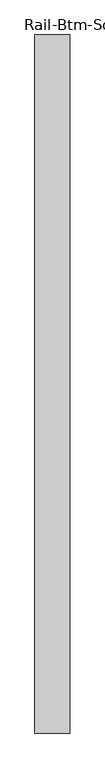
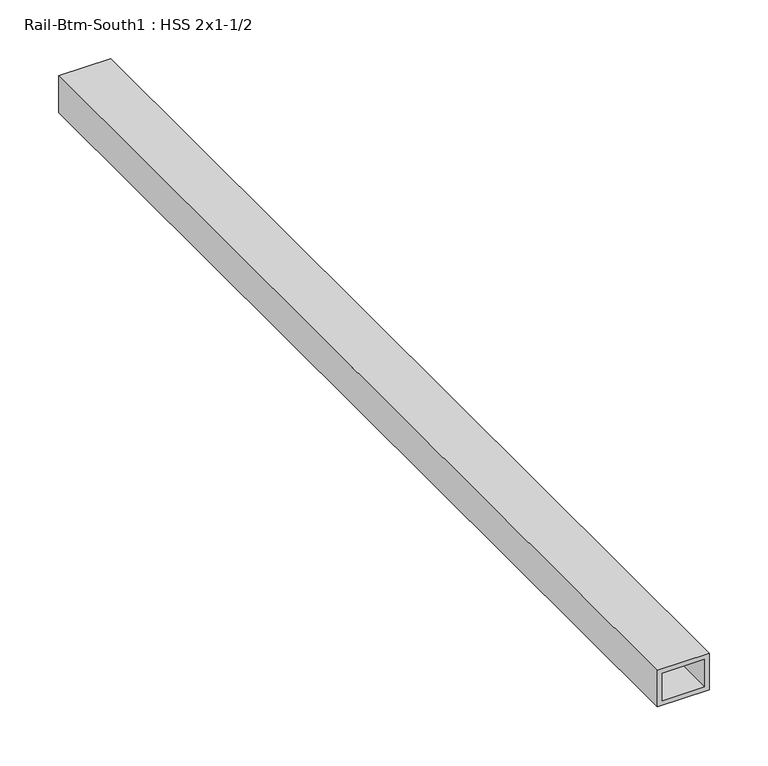
"""IFC4 building model written with IfcOpenShell, lengths in millimetres: proxy geometry, Rail-Btm-South1 : HSS 2x1-1/2."""

from ifc_helpers import new_model, si_unit, frame, origin, place, context, project, spatial, polyline, outline, extrude, source, transform, mapped, element, save


def rail_btm_south1_hss_2x1_1_2_3e8d5585(model_context):
    return source(origin(), model_context, "Body", "SweptSolid", [
        extrude(outline(polyline([(50.8, 587416.6934739), (88.9, 587416.6934739), (88.9, 587365.8934739), (50.8, 587365.8934739), (50.8, 587416.6934739)]), holes=[polyline([(84.1375, 587411.9309739), (55.5625, 587411.9309739), (55.5625, 587370.6559739), (84.1375, 587370.6559739), (84.1375, 587411.9309739)])]), frame((0.0, -536263.6038841, 0.0), z_axis=(0.0, 1.0, 0.0), x_axis=(0.0, 0.0, 1.0)), (0.0, 0.0, 1.0), 1017.5875),
    ])


if __name__ == "__main__":
    model = new_model("IFC4")
    model_context = context("Model", 3, world=origin())
    ifc_project = project(units=[si_unit("LENGTHUNIT", "METRE", prefix="MILLI")], contexts=[model_context])
    site = spatial("IfcSite", under=ifc_project)
    building = spatial("IfcBuilding", under=site)
    placement = place(None, origin())
    rail_btm_south1_hss_2x1_1_2_shape = rail_btm_south1_hss_2x1_1_2_3e8d5585(model_context)
    element("IfcBuildingElementProxy", 1, Name="Rail-Btm-South1 : HSS 2x1-1/2", ObjectType="Rail-Btm-South1 : HSS 2x1-1/2", at=placement, inside=building, context=model_context, shape_type="MappedRepresentation", body=[
        mapped(rail_btm_south1_hss_2x1_1_2_shape, transform((0.0, 0.0, 0.0), x_axis=(1.0, 0.0, 0.0), y_axis=(0.0, 1.0, 0.0), z_axis=(0.0, 0.0, 1.0))),
    ])
    save(model, "model.ifc")

# Revit data of these elements
# Element 1 (IfcBuildingElementProxy, "Rail-Btm-South1 : HSS 2x1-1/2")
#   Materials on its faces: "1-1/2\"X2\" GALV. STL HSS TUBING"
# Materials
#   "1-1/2\"X2\" GALV. STL HSS TUBING": class "Generic", colour RGB 211 211 207, transparency 0, Cost = 0
